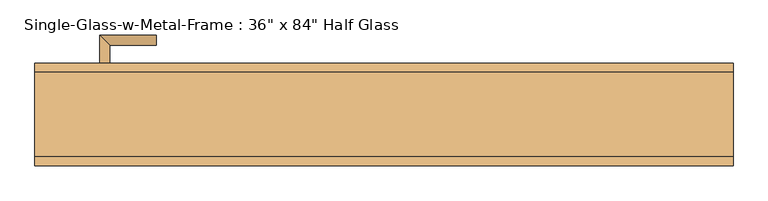
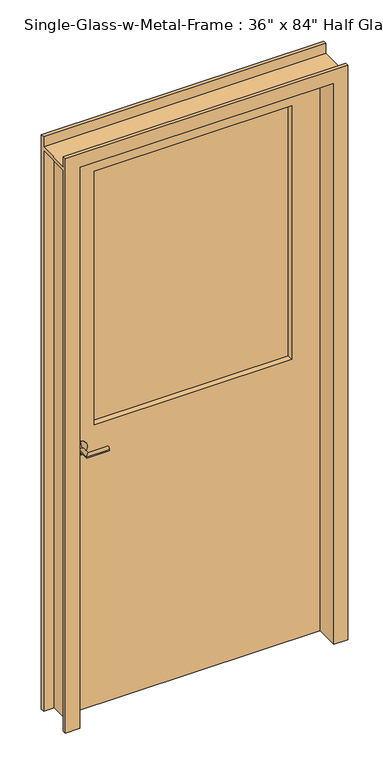
"""IFC4 building model written with IfcOpenShell, lengths in millimetres: door geometry."""

from ifc_helpers import new_model, si_unit, point, frame, origin, place, context, project, spatial, polyline, circle_curve, ellipse_curve, trimmed, outline, extrude, faceted_brep, source, transform, mapped, element, save
from ifc_brep_helpers import plane_surface, cylinder_surface, revolved_surface, advanced_brep


def door_43c3af53(model_context):
    return source(origin(), model_context, "Body", "SolidModel", [
        advanced_brep(
        [(-406.4, 7.9375, 971.55), (-406.4, -0.5511179, 989.45), (-413.9, -0.5511179, 996.95), (-406.4, -0.5511179, 1004.45), (-406.4, 7.9375, 1022.35), (-398.9, -0.5511179, 996.95), (-406.4, 11.1125, 1022.35), (-406.4, 11.1125, 971.55), (-406.4, 11.1125, 996.95), (-413.9, -42.4875, 996.95), (-398.9, -27.4875, 996.95), (-331.4, -42.4875, 996.95), (-331.4, -27.4875, 996.95)],
        [
            (0, 1, circle_curve(frame((-406.4, -28.6667775, 965.1541113), z_axis=(1.0, 0.0, 0.0), x_axis=(0.0, 0.0, 1.0)), 37.1588553)),
            (1, 2, circle_curve(frame((-406.4, -0.5511179, 996.95), z_axis=(0.0, 1.0, 0.0), x_axis=(0.0, 0.0, 1.0)), 7.5)),
            (2, 3, circle_curve(frame((-406.4, -0.5511179, 996.95), z_axis=(0.0, 1.0, 0.0), x_axis=(0.0, 0.0, 1.0)), 7.5)),
            (3, 4, circle_curve(frame((-406.4, -28.6667775, 1028.7458887), z_axis=(1.0, 0.0, 0.0), x_axis=(0.0, 0.0, -1.0)), 37.1588553)),
            (4, 0, circle_curve(frame((-406.4, 7.9375, 996.95), z_axis=(0.0, -1.0, 0.0), x_axis=(0.0, 0.0, 1.0)), 25.4)),
            (3, 5, circle_curve(frame((-406.4, -0.5511179, 996.95), z_axis=(0.0, 1.0, 0.0), x_axis=(0.0, 0.0, 1.0)), 7.5)),
            (5, 1, circle_curve(frame((-406.4, -0.5511179, 996.95), z_axis=(0.0, 1.0, 0.0), x_axis=(0.0, 0.0, 1.0)), 7.5)),
            (0, 4, circle_curve(frame((-406.4, 7.9375, 996.95), z_axis=(0.0, -1.0, 0.0), x_axis=(0.0, 0.0, 1.0)), 25.4)),
            (4, 6),
            (6, 7, circle_curve(frame((-406.4, 11.1125, 996.95), z_axis=(0.0, -1.0, 0.0), x_axis=(0.0, 0.0, 1.0)), 25.4)),
            (7, 0),
            (7, 6, circle_curve(frame((-406.4, 11.1125, 996.95), z_axis=(0.0, -1.0, 0.0), x_axis=(0.0, 0.0, 1.0)), 25.4)),
            (6, 8),
            (8, 7),
            (9, 2),
            (5, 10),
            (10, 9, ellipse_curve(frame((-406.4, -34.9875, 996.95), z_axis=(-0.7071067811864695, 0.7071067811866254, 0.0), x_axis=(0.7071067811866254, 0.7071067811864696, 0.0)), 10.6066017, 7.5)),
            (9, 10, ellipse_curve(frame((-406.4, -34.9875, 996.95), z_axis=(-0.7071067811864695, 0.7071067811866254, 0.0), x_axis=(0.7071067811866254, 0.7071067811864696, 0.0)), 10.6066017, 7.5)),
            (11, 12, circle_curve(frame((-331.4, -34.9875, 996.95), z_axis=(1.0, 0.0, 0.0), x_axis=(0.0, 1.0, 0.0)), 7.5)),
            (12, 11, circle_curve(frame((-331.4, -34.9875, 996.95), z_axis=(1.0, 0.0, 0.0), x_axis=(0.0, 1.0, 0.0)), 7.5)),
            (10, 12),
            (11, 9),
        ],
        [
            revolved_surface(trimmed(ellipse_curve(frame((-406.4, -28.6667775, 1028.7458887), z_axis=(1.0, 0.0, 0.0), x_axis=(0.0, 0.0, -1.0)), 37.1588553, 37.1588553), [point((-406.4, -1.5875, 1003.3))], [point((-406.4, 7.9375, 1022.35))], True, "CARTESIAN"), (-406.4, -1.5875, 996.95), (0.0, 1.0, 0.0)),
            cylinder_surface(frame((-406.4, -1.5875, 996.95), z_axis=(0.0, 1.0, 0.0), x_axis=(0.0, 0.0, 1.0)), 25.4),
            plane_surface(frame((-406.4, 11.1125, 996.95), z_axis=(0.0, 1.0, 0.0), x_axis=(0.0, 0.0, 1.0))),
            cylinder_surface(frame((-406.4, 3.1125, 996.95), z_axis=(0.0, 1.0, 0.0), x_axis=(1.0, 0.0, 0.0)), 7.5),
            plane_surface(frame((-331.4, -34.9875, 996.95), z_axis=(1.0, 0.0, 0.0), x_axis=(0.0, 0.0, 1.0))),
            cylinder_surface(frame((-406.4, -34.9875, 996.95), z_axis=(-1.0, 0.0, 0.0), x_axis=(0.0, 1.0, 0.0)), 7.5),
        ],
        [
            (0, [[1, 2, 3, 4, 5]]),
            (0, [[-4, 6, 7, -1, 8]]),
            (1, [[9, 10, 11, -5]]),
            (1, [[-11, 12, -9, -8]]),
            (2, [[13, 14, -10]]),
            (2, [[-14, -13, -12]]),
            (3, [[15, -2, -7, 16, 17]]),
            (3, [[-16, -6, -3, -15, 18]]),
            (4, [[19, 20]]),
            (5, [[21, -19, 22, -17]]),
            (5, [[-22, -20, -21, -18]]),
        ],
    ),
        advanced_brep(
        [(-406.4, 65.0875, 971.55), (-406.4, 65.0875, 1022.35), (-406.4, 73.5761179, 1004.45), (-413.9, 73.5761179, 996.95), (-406.4, 73.5761179, 989.45), (-398.9, 73.5761179, 996.95), (-406.4, 61.9125, 971.55), (-406.4, 61.9125, 1022.35), (-406.4, 61.9125, 996.95), (-413.9, 115.5125, 996.95), (-398.9, 100.5125, 996.95), (-331.4, 115.5125, 996.95), (-331.4, 100.5125, 996.95)],
        [
            (0, 1, circle_curve(frame((-406.4, 65.0875, 996.95), z_axis=(0.0, 1.0, 0.0), x_axis=(0.0, 0.0, 1.0)), 25.4)),
            (1, 2, circle_curve(frame((-406.4, 101.6917775, 1028.7458887), z_axis=(1.0, 0.0, 0.0), x_axis=(0.0, 0.0, -1.0)), 37.1588553)),
            (2, 3, circle_curve(frame((-406.4, 73.5761179, 996.95), z_axis=(0.0, -1.0, 0.0), x_axis=(0.0, 0.0, 1.0)), 7.5)),
            (3, 4, circle_curve(frame((-406.4, 73.5761179, 996.95), z_axis=(0.0, -1.0, 0.0), x_axis=(0.0, 0.0, 1.0)), 7.5)),
            (4, 0, circle_curve(frame((-406.4, 101.6917775, 965.1541113), z_axis=(1.0, 0.0, 0.0), x_axis=(0.0, 0.0, 1.0)), 37.1588553)),
            (1, 0, circle_curve(frame((-406.4, 65.0875, 996.95), z_axis=(0.0, 1.0, 0.0), x_axis=(0.0, 0.0, 1.0)), 25.4)),
            (4, 5, circle_curve(frame((-406.4, 73.5761179, 996.95), z_axis=(0.0, -1.0, 0.0), x_axis=(0.0, 0.0, 1.0)), 7.5)),
            (5, 2, circle_curve(frame((-406.4, 73.5761179, 996.95), z_axis=(0.0, -1.0, 0.0), x_axis=(0.0, 0.0, 1.0)), 7.5)),
            (0, 6),
            (6, 7, circle_curve(frame((-406.4, 61.9125, 996.95), z_axis=(0.0, 1.0, 0.0), x_axis=(0.0, 0.0, 1.0)), 25.4)),
            (7, 1),
            (7, 6, circle_curve(frame((-406.4, 61.9125, 996.95), z_axis=(0.0, 1.0, 0.0), x_axis=(0.0, 0.0, 1.0)), 25.4)),
            (6, 8),
            (8, 7),
            (9, 10, ellipse_curve(frame((-406.4, 108.0125, 996.95), z_axis=(-0.7071067811864695, -0.7071067811866254, 0.0), x_axis=(0.7071067811866254, -0.7071067811864696, 0.0)), 10.6066017, 7.5)),
            (10, 5),
            (3, 9),
            (10, 9, ellipse_curve(frame((-406.4, 108.0125, 996.95), z_axis=(-0.7071067811864695, -0.7071067811866254, 0.0), x_axis=(0.7071067811866254, -0.7071067811864696, 0.0)), 10.6066017, 7.5)),
            (11, 12, circle_curve(frame((-331.4, 108.0125, 996.95), z_axis=(1.0, 0.0, 0.0), x_axis=(0.0, -1.0, 0.0)), 7.5)),
            (12, 11, circle_curve(frame((-331.4, 108.0125, 996.95), z_axis=(1.0, 0.0, 0.0), x_axis=(0.0, -1.0, 0.0)), 7.5)),
            (9, 11),
            (12, 10),
        ],
        [
            revolved_surface(trimmed(ellipse_curve(frame((-406.4, 101.6917775, 1028.7458887), z_axis=(-1.0, 0.0, 0.0), x_axis=(0.0, 0.0, -1.0)), 37.1588553, 37.1588553), [point((-406.4, 74.6125, 1003.3))], [point((-406.4, 65.0875, 1022.35))], True, "CARTESIAN"), (-406.4, 74.6125, 996.95), (0.0, -1.0, 0.0)),
            cylinder_surface(frame((-406.4, 74.6125, 996.95), z_axis=(0.0, -1.0, 0.0), x_axis=(0.0, 0.0, 1.0)), 25.4),
            plane_surface(frame((-406.4, 61.9125, 996.95), z_axis=(0.0, -1.0, 0.0), x_axis=(0.0, 0.0, 1.0))),
            cylinder_surface(frame((-406.4, 69.9125, 996.95), z_axis=(0.0, -1.0, 0.0), x_axis=(1.0, 0.0, 0.0)), 7.5),
            plane_surface(frame((-331.4, 108.0125, 996.95), z_axis=(1.0, 0.0, 0.0), x_axis=(0.0, 0.0, 1.0))),
            cylinder_surface(frame((-406.4, 108.0125, 996.95), z_axis=(-1.0, 0.0, 0.0), x_axis=(0.0, -1.0, 0.0)), 7.5),
        ],
        [
            (0, [[1, 2, 3, 4, 5]]),
            (0, [[6, -5, 7, 8, -2]]),
            (1, [[-1, 9, 10, 11]]),
            (1, [[-6, -11, 12, -9]]),
            (2, [[-10, 13, 14]]),
            (2, [[-12, -14, -13]]),
            (3, [[15, 16, -7, -4, 17]]),
            (3, [[18, -17, -3, -8, -16]]),
            (4, [[19, 20]]),
            (5, [[-15, 21, -20, 22]]),
            (5, [[-18, -22, -19, -21]]),
        ],
    ),
        extrude(outline(polyline([(355.6, 33.3375), (-355.6, 33.3375), (-355.6, 39.6875), (355.6, 39.6875), (355.6, 33.3375)])), frame((0.0, 0.0, 1066.8), z_axis=(0.0, 0.0, 1.0), x_axis=(1.0, 0.0, 0.0)), (0.0, 0.0, 1.0), 965.2),
        extrude(outline(polyline([(2133.6, 457.2), (2133.6, -457.2), (0.0, -457.2), (0.0, 457.2), (2133.6, 457.2)]), holes=[polyline([(2032.0, -355.6), (2032.0, 355.6), (1066.8, 355.6), (1066.8, -355.6), (2032.0, -355.6)])]), frame((0.0, 11.1125, 0.0), z_axis=(0.0, 1.0, 0.0), x_axis=(0.0, 0.0, 1.0)), (0.0, 0.0, 1.0), 50.8),
        faceted_brep([(-469.9, 61.9125, 0.0), (-508.0, 61.9125, 0.0), (-508.0, 74.6125, 0.0), (-457.2, 74.6125, 0.0), (-457.2, -74.6125, 0.0), (-508.0, -74.6125, 0.0), (-508.0, -61.9125, 0.0), (-469.9, -61.9125, 0.0), (-469.9, 61.9125, 2133.6), (-508.0, 61.9125, 2133.6), (-508.0, -61.9125, 2133.6), (-508.0, -74.6125, 2184.4), (-508.0, -61.9125, 2184.4), (-508.0, -61.9125, 2146.3), (-508.0, 61.9125, 2146.3), (-508.0, 61.9125, 2184.4), (-508.0, 74.6125, 2184.4), (508.0, 74.6125, 2184.4), (508.0, 74.6125, 0.0), (457.2, 74.6125, 0.0), (457.2, 74.6125, 2133.6), (-457.2, 74.6125, 2133.6), (-457.2, -74.6125, 2133.6), (457.2, -74.6125, 2133.6), (457.2, -74.6125, 0.0), (508.0, -74.6125, 0.0), (508.0, -74.6125, 2184.4), (-469.9, -61.9125, 2133.6), (469.9, 61.9125, 0.0), (469.9, -61.9125, 0.0), (508.0, -61.9125, 0.0), (508.0, 61.9125, 0.0), (508.0, -61.9125, 2146.3), (508.0, -61.9125, 2184.4), (508.0, -61.9125, 2133.6), (508.0, 61.9125, 2133.6), (508.0, 61.9125, 2184.4), (508.0, 61.9125, 2146.3), (469.9, -61.9125, 2133.6), (469.9, 61.9125, 2133.6)], [[[0, 1, 2, 3, 4, 5, 6, 7]], [[1, 0, 8, 9]], [[2, 1, 9, 10, 6, 5, 11, 12, 13, 14, 15, 16]], [[3, 2, 16, 17, 18, 19, 20, 21]], [[4, 3, 21, 22]], [[5, 4, 22, 23, 24, 25, 26, 11]], [[7, 6, 10, 27]], [[0, 7, 27, 8]], [[19, 24, 23, 20]], [[28, 29, 30, 25, 24, 19, 18, 31]], [[32, 33, 26, 25, 30, 34, 35, 31, 18, 17, 36, 37]], [[30, 29, 38, 34]], [[28, 31, 35, 39]], [[29, 28, 39, 38]], [[33, 32, 13, 12]], [[26, 33, 12, 11]], [[10, 9, 8, 27]], [[22, 21, 20, 23]], [[35, 34, 38, 39]], [[36, 17, 16, 15]], [[37, 36, 15, 14]], [[32, 37, 14, 13]]]),
    ])


if __name__ == "__main__":
    model = new_model("IFC4")
    model_context = context("Model", 3, world=origin())
    ifc_project = project(units=[si_unit("LENGTHUNIT", "METRE", prefix="MILLI")], contexts=[model_context])
    site = spatial("IfcSite", under=ifc_project)
    building = spatial("IfcBuilding", under=site)
    placement = place(None, origin())
    door_shape = door_43c3af53(model_context)
    element("IfcDoor", 1, ObjectType="Single-Glass-w-Metal-Frame : 36\" x 84\" Half Glass", at=placement, inside=building, context=model_context, shape_type="MappedRepresentation", body=[
        mapped(door_shape, transform((0.0, 0.0, 0.0), x_axis=(1.0, 0.0, 0.0), y_axis=(0.0, 1.0, 0.0), z_axis=(0.0, 0.0, 1.0))),
    ])
    save(model, "model.ifc")

# Revit data of these elements
# Type "Single-Glass-w-Metal-Frame : 36\" x 84\" Half Glass"
#   Type Mark = "15"
#   Construction Type Id = "MDOOR"
#   Assembly Code = "C1020"
#   Analytic Construction = "Metal"
#   Thickness = 0' - 2"
#   Thermal Resistance (R) = 1.5338 (h·ft²·°F)/BTU
#   Half Width Neg = -1' - 8"
#   Half Width = 1' - 8"
#   Frame Width = 0' - 2"
#   Frame Thickness = 0' - 0 1/2"
#   Frame Head Heigth = 0' - 2"
#   Heat Transfer Coefficient (U) = 0.651978 BTU/(h·ft²·°F)
#   Height = 7' - 0"
#   Rail Width - Base = 3' - 6"
#   Rail Width - Top = 0' - 4"
#   Stile Width - Hinge = 0' - 4"
#   Stile Width - Latch = 0' - 4"
#   Width = 3' - 0"
#   Define Thermal Properties by = 1
#   Define Thermal Properties by = 1
#   Glazing Material = Glass
#   Door Material = Door - Panel
#   Frame Material = Door - Frame
#   Visual Light Transmittance = 0
#   Solar Heat Gain Coefficient = 0
#   Function = (empty or 0)
#   Wall Closure = (empty or 0)
# Element 1 (IfcDoor, "Single-Glass-w-Metal-Frame : 36\" x 84\" Half Glass")
#   Materials on its faces: "Metal - Aluminium", "Door - Frame", "Door - Panel", "Glass"
# Materials
#   "Glass": class "Glass", colour RGB 0 128 192, transparency 0.75, Description = "Soda Lime Glass", Cost = 0
#   "Door - Panel": class "Wood", colour RGB 210 159 95, transparency 0
#   "Door - Frame": class "Miscellaneous", colour RGB 118 70 51, transparency 0
#   "Metal - Aluminium": class "Unassigned", colour RGB 247 247 247, transparency 0
